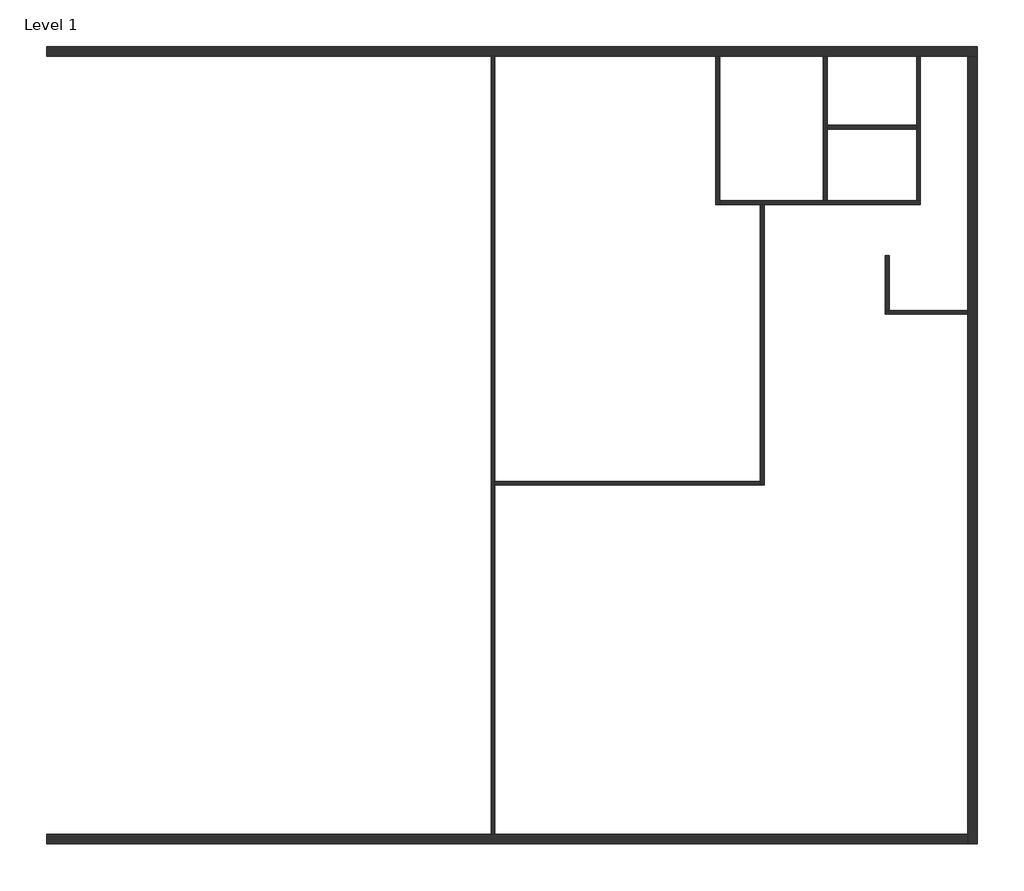
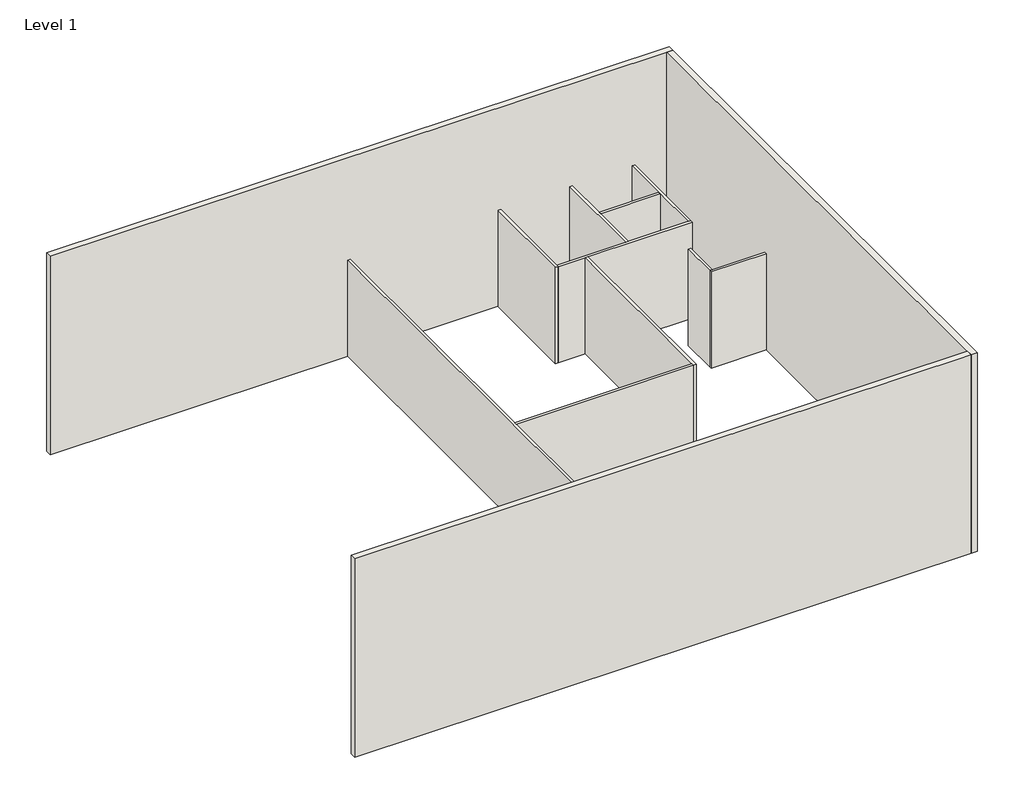
# One storey: 13 walls.
"""IFC4 building model written with IfcOpenShell, lengths in millimetres."""

from ifc_helpers import new_model, si_unit, origin, origin_with_axes, place, context, project, spatial, polyline, outline, extrude, faceted_brep, element, save

model = new_model("IFC4")

# Units and contexts
model_context = context("Model", 3, world=origin())
ifc_project = project(units=[si_unit("LENGTHUNIT", "METRE", prefix="MILLI")], contexts=[model_context])

# Site, building, storey
site = spatial("IfcSite", under=ifc_project)
building = spatial("IfcBuilding", under=site)
storey = spatial("IfcBuildingStorey", under=building, Name="Level 1", Elevation=0.0)

# Walls
placement = place(None, origin())
element("IfcWall", 1, ObjectType="Generic - 12\"", at=placement, inside=storey, context=model_context, shape_type="Brep", body=[
    faceted_brep([(-11486.7262822, 13482.5120281, 0.0), (2775.3737178, 13482.5120281, 0.0), (2902.3737178, 13482.5120281, 0.0), (9988.9737178, 13482.5120281, 0.0), (10115.9737178, 13482.5120281, 0.0), (13430.6737178, 13482.5120281, 0.0), (13557.6737178, 13482.5120281, 0.0), (16427.8737178, 13482.5120281, 0.0), (16554.8737178, 13482.5120281, 0.0), (18078.8737178, 13482.5120281, 0.0), (18383.6737178, 13482.5120281, 0.0), (18383.6737178, 13482.5120281, 10058.4), (18078.8737178, 13482.5120281, 10058.4), (-11486.7262822, 13482.5120281, 10058.4), (-11486.7262822, 13787.3120281, 0.0), (-11486.7262822, 13787.3120281, 10058.4), (18383.6737178, 13787.3120281, 10058.4), (18383.6737178, 13787.3120281, 0.0)], [[[0, 1, 2, 3, 4, 5, 6, 7, 8, 9, 10, 11, 12, 13]], [[14, 15, 16, 17]], [[10, 9, 8, 7, 6, 5, 4, 3, 2, 1, 0, 14, 17]], [[13, 12, 11, 16, 15]], [[0, 13, 15, 14]], [[11, 10, 17, 16]]]),
])
element("IfcWall", 2, ObjectType="Generic - 12\"", at=placement, inside=storey, context=model_context, shape_type="Brep", body=[
    faceted_brep([(18078.8737178, 13482.5120281, 0.0), (18078.8737178, 5316.4120281, 0.0), (18078.8737178, 5189.4120281, 0.0), (18078.8737178, -11511.0879719, 0.0), (18078.8737178, -11815.8879719, 0.0), (18078.8737178, -11815.8879719, 10058.4), (18078.8737178, -11511.0879719, 10058.4), (18078.8737178, 13482.5120281, 10058.4), (18383.6737178, 13482.5120281, 0.0), (18383.6737178, 13482.5120281, 10058.4), (18383.6737178, -11815.8879719, 10058.4), (18383.6737178, -11815.8879719, 0.0)], [[[0, 1, 2, 3, 4, 5, 6, 7]], [[8, 9, 10, 11]], [[4, 3, 2, 1, 0, 8, 11]], [[7, 6, 5, 10, 9]], [[0, 7, 9, 8]], [[5, 4, 11, 10]]]),
])
element("IfcWall", 3, ObjectType="Generic - 12\"", at=placement, inside=storey, context=model_context, shape_type="Brep", body=[
    faceted_brep([(18078.8737178, -11511.0879719, 0.0), (2902.3737178, -11511.0879719, 0.0), (2775.3737178, -11511.0879719, 0.0), (-11486.7262822, -11511.0879719, 0.0), (-11486.7262822, -11511.0879719, 10058.4), (18078.8737178, -11511.0879719, 10058.4), (18078.8737178, -11815.8879719, 0.0), (18078.8737178, -11815.8879719, 10058.4), (-11486.7262822, -11815.8879719, 10058.4), (-11486.7262822, -11815.8879719, 0.0)], [[[0, 1, 2, 3, 4, 5]], [[6, 7, 8, 9]], [[3, 2, 1, 0, 6, 9]], [[4, 3, 9, 8]], [[5, 4, 8, 7]], [[0, 5, 7, 6]]]),
])
element("IfcWall", 4, ObjectType="Generic - 5\"", at=placement, inside=storey, context=model_context, shape_type="Brep", body=[
    faceted_brep([(2902.3737178, -11511.0879719, 0.0), (2902.3737178, -296.9879719, 0.0), (2902.3737178, -169.9879719, 0.0), (2902.3737178, 13482.5120281, 0.0), (2902.3737178, 13482.5120281, 4876.8), (2902.3737178, -169.9879719, 4876.8), (2902.3737178, -296.9879719, 4876.8), (2902.3737178, -11511.0879719, 4876.8), (2775.3737178, -11511.0879719, 0.0), (2775.3737178, -11511.0879719, 4876.8), (2775.3737178, 13482.5120281, 4876.8), (2775.3737178, 13482.5120281, 0.0)], [[[0, 1, 2, 3, 4, 5, 6, 7]], [[8, 9, 10, 11]], [[3, 2, 1, 0, 8, 11]], [[7, 6, 5, 4, 10, 9]], [[4, 3, 11, 10]], [[0, 7, 9, 8]]]),
])
element("IfcWall", 5, ObjectType="Generic - 5\"", at=placement, inside=storey, context=model_context, shape_type="Brep", body=[
    faceted_brep([(9988.9737178, 13482.5120281, 0.0), (9988.9737178, 8707.3120281, 0.0), (9988.9737178, 8707.3120281, 4876.8), (9988.9737178, 13482.5120281, 4876.8), (10115.9737178, 13482.5120281, 0.0), (10115.9737178, 13482.5120281, 4876.8), (10115.9737178, 8834.3120281, 4876.8), (10115.9737178, 8707.3120281, 4876.8), (10115.9737178, 8707.3120281, 0.0), (10115.9737178, 8834.3120281, 0.0)], [[[0, 1, 2, 3]], [[4, 5, 6, 7, 8, 9]], [[1, 0, 4, 9, 8]], [[3, 2, 7, 6, 5]], [[0, 3, 5, 4]], [[2, 1, 8, 7]]]),
])
element("IfcWall", 6, ObjectType="Generic - 5\"", at=placement, inside=storey, context=model_context, shape_type="Brep", body=[
    faceted_brep([(10115.9737178, 8707.3120281, 0.0), (11411.3737178, 8707.3120281, 0.0), (11538.3737178, 8707.3120281, 0.0), (16554.8737178, 8707.3120281, 0.0), (16554.8737178, 8707.3120281, 4876.8), (11538.3737178, 8707.3120281, 4876.8), (11411.3737178, 8707.3120281, 4876.8), (10115.9737178, 8707.3120281, 4876.8), (10115.9737178, 8834.3120281, 0.0), (10115.9737178, 8834.3120281, 4876.8), (13430.6737178, 8834.3120281, 4876.8), (13557.6737178, 8834.3120281, 4876.8), (16427.8737178, 8834.3120281, 4876.8), (16554.8737178, 8834.3120281, 4876.8), (16554.8737178, 8834.3120281, 0.0), (16427.8737178, 8834.3120281, 0.0), (13557.6737178, 8834.3120281, 0.0), (13430.6737178, 8834.3120281, 0.0)], [[[0, 1, 2, 3, 4, 5, 6, 7]], [[8, 9, 10, 11, 12, 13, 14, 15, 16, 17]], [[3, 2, 1, 0, 8, 17, 16, 15, 14]], [[7, 6, 5, 4, 13, 12, 11, 10, 9]], [[0, 7, 9, 8]], [[4, 3, 14, 13]]]),
])
element("IfcWall", 7, ObjectType="Generic - 5\"", at=placement, inside=storey, context=model_context, shape_type="Brep", body=[
    faceted_brep([(16554.8737178, 8834.3120281, 0.0), (16554.8737178, 13482.5120281, 0.0), (16554.8737178, 13482.5120281, 4876.8), (16554.8737178, 8834.3120281, 4876.8), (16427.8737178, 8834.3120281, 0.0), (16427.8737178, 8834.3120281, 4876.8), (16427.8737178, 11139.3620281, 4876.8), (16427.8737178, 11266.3620281, 4876.8), (16427.8737178, 13482.5120281, 4876.8), (16427.8737178, 13482.5120281, 0.0), (16427.8737178, 11266.3620281, 0.0), (16427.8737178, 11139.3620281, 0.0)], [[[0, 1, 2, 3]], [[4, 5, 6, 7, 8, 9, 10, 11]], [[1, 0, 4, 11, 10, 9]], [[3, 2, 8, 7, 6, 5]], [[0, 3, 5, 4]], [[2, 1, 9, 8]]]),
])
element("IfcWall", 8, ObjectType="Generic - 5\"", at=placement, inside=storey, context=model_context, shape_type="Brep", body=[
    faceted_brep([(13430.6737178, 13482.5120281, 0.0), (13430.6737178, 8834.3120281, 0.0), (13430.6737178, 8834.3120281, 4876.8), (13430.6737178, 13482.5120281, 4876.8), (13557.6737178, 13482.5120281, 0.0), (13557.6737178, 13482.5120281, 4876.8), (13557.6737178, 11266.3620281, 4876.8), (13557.6737178, 11139.3620281, 4876.8), (13557.6737178, 8834.3120281, 4876.8), (13557.6737178, 8834.3120281, 0.0), (13557.6737178, 11139.3620281, 0.0), (13557.6737178, 11266.3620281, 0.0)], [[[0, 1, 2, 3]], [[4, 5, 6, 7, 8, 9, 10, 11]], [[1, 0, 4, 11, 10, 9]], [[3, 2, 8, 7, 6, 5]], [[0, 3, 5, 4]], [[2, 1, 9, 8]]]),
])
element("IfcWall", 9, ObjectType="Generic - 5\"", at=placement, inside=storey, context=model_context, shape_type="SweptSolid", body=[
    extrude(outline(polyline([(13557.6737178, 11266.3620281), (16427.8737178, 11266.3620281), (16427.8737178, 11139.3620281), (13557.6737178, 11139.3620281), (13557.6737178, 11266.3620281)])), origin_with_axes(), (0.0, 0.0, 1.0), 4876.8),
])
element("IfcWall", 10, ObjectType="Generic - 5\"", at=placement, inside=storey, context=model_context, shape_type="Brep", body=[
    faceted_brep([(18078.8737178, 5316.4120281, 0.0), (15551.5737178, 5316.4120281, 0.0), (15424.5737178, 5316.4120281, 0.0), (15424.5737178, 5316.4120281, 4876.8), (15551.5737178, 5316.4120281, 4876.8), (18078.8737178, 5316.4120281, 4876.8), (18078.8737178, 5189.4120281, 0.0), (18078.8737178, 5189.4120281, 4876.8), (15424.5737178, 5189.4120281, 4876.8), (15424.5737178, 5189.4120281, 0.0)], [[[0, 1, 2, 3, 4, 5]], [[6, 7, 8, 9]], [[2, 1, 0, 6, 9]], [[5, 4, 3, 8, 7]], [[0, 5, 7, 6]], [[3, 2, 9, 8]]]),
])
element("IfcWall", 11, ObjectType="Generic - 5\"", at=placement, inside=storey, context=model_context, shape_type="SweptSolid", body=[
    extrude(outline(polyline([(15551.5737178, 7081.7120281), (15551.5737178, 5316.4120281), (15424.5737178, 5316.4120281), (15424.5737178, 7081.7120281), (15551.5737178, 7081.7120281)])), origin_with_axes(), (0.0, 0.0, 1.0), 4876.8),
])
element("IfcWall", 12, ObjectType="Generic - 5\"", at=placement, inside=storey, context=model_context, shape_type="Brep", body=[
    faceted_brep([(11411.3737178, 8707.3120281, 0.0), (11411.3737178, -169.9879719, 0.0), (11411.3737178, -296.9879719, 0.0), (11411.3737178, -296.9879719, 4876.8), (11411.3737178, -169.9879719, 4876.8), (11411.3737178, 8707.3120281, 4876.8), (11538.3737178, 8707.3120281, 0.0), (11538.3737178, 8707.3120281, 4876.8), (11538.3737178, -296.9879719, 4876.8), (11538.3737178, -296.9879719, 0.0)], [[[0, 1, 2, 3, 4, 5]], [[6, 7, 8, 9]], [[2, 1, 0, 6, 9]], [[5, 4, 3, 8, 7]], [[0, 5, 7, 6]], [[3, 2, 9, 8]]]),
])
element("IfcWall", 13, ObjectType="Generic - 5\"", at=placement, inside=storey, context=model_context, shape_type="SweptSolid", body=[
    extrude(outline(polyline([(2902.3737178, -169.9879719), (11411.3737178, -169.9879719), (11411.3737178, -296.9879719), (2902.3737178, -296.9879719), (2902.3737178, -169.9879719)])), origin_with_axes(), (0.0, 0.0, 1.0), 4876.8),
])

save(model, "model.ifc")

# Revit data of these elements
# Project information
#   Project Issue Date = "Issue Date"
#   Project Status = "Project Status"
#   Client Name = "Owner"
#   Project Address = "Enter address here"
#   Project Name = "Project Name"
#   Project Number = "Project Number"
# Grids (mm)
#   "1": line (-18801.926, 15817.913) -> (-18801.926, -14896.109)
#   "2": line (-11486.726, 15817.913) -> (-11486.726, -14896.109)
#   "3": line (-4171.526, 15817.913) -> (-4171.526, -14896.109)
#   "4": line (3143.674, 15817.913) -> (3143.674, -14896.109)
#   "5": line (10458.874, 15817.913) -> (10458.874, -14896.109)
#   "6": line (17774.074, 15817.913) -> (17774.074, -14896.109)
#   "A": line (23913.763, 13177.712) -> (-22245.007, 13177.712)
#   "B": line (23913.763, 5862.512) -> (-22245.007, 5862.512)
#   "C": line (23913.763, -2671.888) -> (-22245.007, -2671.888)
#   "D": line (23913.763, -11206.288) -> (-22245.007, -11206.288)
# Type "Generic - 12\""
#   Assembly Code = "B2010"
#   Layers, outside or top first: 1' - 0" no material (function 1)
# Type "Generic - 5\""
#   Assembly Code = "B2010"
#   Layers, outside or top first: 0' - 5" no material (function 1)
# Elements 1, 2, 3 (IfcWall, "Generic - 12\"")
#   Top Offset = 0' - 0"
#   Base Offset = 0' - 0"
#   wall height = 33' - 0"
#   Phase Created = New Construction
#   Base Constraint = Level 1
#   Top Constraint = Parapet
#   Materials on its faces: "Default Wall"
# Elements 4, 5, 6, 7, 8, 9, 10, 11, 12, 13 (IfcWall, "Generic - 5\"")
#   Top Offset = 0' - 0"
#   Base Offset = 0' - 0"
#   wall height = 16' - 0"
#   Phase Created = New Construction
#   Base Constraint = Level 1
#   Top Constraint = Level 2
#   Materials on its faces: "Default Wall"
# Materials
#   "Default Wall": class "Miscellaneous", colour RGB 127 127 127, transparency 0, Cost = 0
